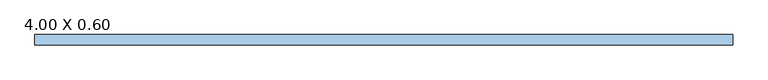
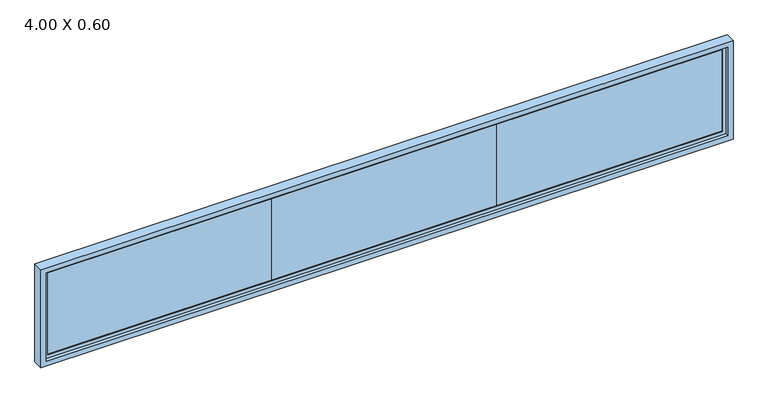
"""IFC4 building model written with IfcOpenShell, lengths in millimetres: window geometry, .CC_ND 300_JANELA FIXA_VIDRO : 4.00 X 0.60."""

from ifc_helpers import new_model, si_unit, frame, origin, place, context, project, spatial, polyline, outline, extrude, source, transform, mapped, element, save


def window_4_00_x_0_60_0b555443(model_context):
    return source(origin(), model_context, "Body", "SweptSolid", [
        extrude(outline(polyline([(650.0, -4.0), (650.0, 4.0), (1950.0, 4.0), (1950.0, -4.0), (650.0, -4.0)])), frame((0.0, 0.0, 1550.0), z_axis=(0.0, 0.0, 1.0), x_axis=(1.0, 0.0, 0.0)), (0.0, 0.0, 1.0), 500.0),
        extrude(outline(polyline([(-650.0, -4.0), (-650.0, 4.0), (650.0, 4.0), (650.0, -4.0), (-650.0, -4.0)])), frame((0.0, 0.0, 1550.0), z_axis=(0.0, 0.0, 1.0), x_axis=(1.0, 0.0, 0.0)), (0.0, 0.0, 1.0), 500.0),
        extrude(outline(polyline([(-1950.0, -4.0), (-1950.0, 4.0), (-650.0, 4.0), (-650.0, -4.0), (-1950.0, -4.0)])), frame((0.0, 0.0, 1550.0), z_axis=(0.0, 0.0, 1.0), x_axis=(1.0, 0.0, 0.0)), (0.0, 0.0, 1.0), 500.0),
        extrude(outline(polyline([(1530.0, 1970.0), (2070.0, 1970.0), (2070.0, -1970.0), (1530.0, -1970.0), (1530.0, 1970.0)]), holes=[polyline([(2050.0, 1950.0), (1550.0, 1950.0), (1550.0, -1950.0), (2050.0, -1950.0), (2050.0, 1950.0)])]), frame((0.0, -10.0, 0.0), z_axis=(0.0, 1.0, 0.0), x_axis=(0.0, 0.0, 1.0)), (0.0, 0.0, 1.0), 20.0),
        extrude(outline(polyline([(1500.0, 2000.0), (2100.0, 2000.0), (2100.0, -2000.0), (1500.0, -2000.0), (1500.0, 2000.0)]), holes=[polyline([(2070.0, 1970.0), (1530.0, 1970.0), (1530.0, -1970.0), (2070.0, -1970.0), (2070.0, 1970.0)])]), frame((0.0, -30.0, 0.0), z_axis=(0.0, 1.0, 0.0), x_axis=(0.0, 0.0, 1.0)), (0.0, 0.0, 1.0), 60.0),
    ])


if __name__ == "__main__":
    model = new_model("IFC4")
    model_context = context("Model", 3, world=origin())
    ifc_project = project(units=[si_unit("LENGTHUNIT", "METRE", prefix="MILLI")], contexts=[model_context])
    site = spatial("IfcSite", under=ifc_project)
    building = spatial("IfcBuilding", under=site)
    placement = place(None, origin())
    window_4_00_x_0_60_shape = window_4_00_x_0_60_0b555443(model_context)
    element("IfcWindow", 1, ObjectType=".CC_ND 300_JANELA FIXA_VIDRO : 4.00 X 0.60", at=placement, inside=building, context=model_context, shape_type="MappedRepresentation", body=[
        mapped(window_4_00_x_0_60_shape, transform((0.0, 0.0, 0.0), x_axis=(1.0, 0.0, 0.0), y_axis=(0.0, 1.0, 0.0), z_axis=(0.0, 0.0, 1.0))),
    ])
    save(model, "model.ifc")

# Revit data of these elements
# Type ".CC_ND 300_JANELA FIXA_VIDRO : 4.00 X 0.60"
#   Type Mark = "60"
#   Largura total vidro [instance default] = 0.90 m
#   Largura Painel [instance default] = 0.02 m
#   Largura Esquadria [instance default] = 0.06 m
#   Espessuras [instance default] = 0.05 m
#   Espessura Vidro [instance default] = 0.008 m
#   Espessura Painel [instance default] = 0.02 m
#   Espessura Esquadria [instance default] = 0.03 m
#   Height = 0.60 m
#   Altura-padrão do peitoril = 1.50 m
#   Width = 4.00 m
#   Vidro = .VIDRO GENÉRICO
#   Esquadria = .ALUMÍNIO COM PINTURA ELETROSTÁTICA BRANCA
#   Wall Closure = (empty or 0)
# Element 1 (IfcWindow, ".CC_ND 300_JANELA FIXA_VIDRO : 4.00 X 0.60")
#   Materials on its faces: ".ALUMÍNIO COM PINTURA ELETROSTÁTICA BRANCA", ".VIDRO GENÉRICO"
# Materials
#   ".VIDRO GENÉRICO": class ".CC_VIDRO", colour RGB 0 128 192, transparency 0.9, Description = "Vidro comum", Cost = 0
#   ".ALUMÍNIO COM PINTURA ELETROSTÁTICA BRANCA": class "CC_METAIS", colour RGB 241 241 241, transparency 0, Cost = 0
